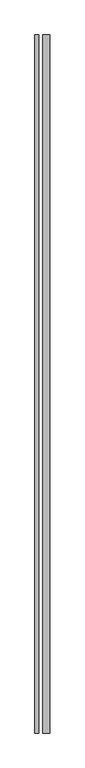
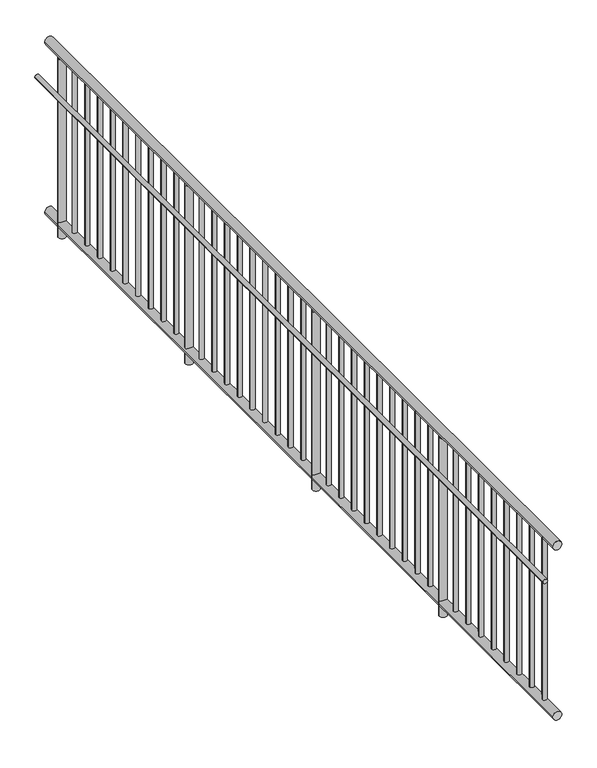
"""IFC4 building model written with IfcOpenShell, lengths in millimetres: railing geometry."""

from ifc_helpers import new_model, si_unit, point, frame, frame_2d, origin, place, context, project, spatial, circle_curve, trimmed, segment, composite_curve, outline, extrude, source, transform, mapped, element, save


def railing_ee1e5d7c(model_context):
    return source(origin(), model_context, "Body", "SweptSolid", [
        extrude(outline(composite_curve([segment(trimmed(circle_curve(frame_2d((4474.6, -1025.274449)), 25.4), [point((4474.6, -999.874449))], [point((4474.6, -1050.674449))], False, "CARTESIAN"), True, "CONTINUOUS"), segment(trimmed(circle_curve(frame_2d((4474.6, -1025.274449)), 25.4), [point((4474.6, -1050.674449))], [point((4474.6, -999.874449))], False, "CARTESIAN"), True, "CONTINUOUS")], self_intersect=False)), frame((0.0, -6784.1965465, 0.0), z_axis=(0.0, 1.0, 0.0), x_axis=(0.0, 0.0, 1.0)), (0.0, 0.0, 1.0), 4890.8),
        extrude(outline(composite_curve([segment(trimmed(circle_curve(frame_2d((4287.3, -1092.274449)), 12.7), [point((4287.3, -1079.574449))], [point((4287.3, -1104.974449))], False, "CARTESIAN"), True, "CONTINUOUS"), segment(trimmed(circle_curve(frame_2d((4287.3, -1092.274449)), 12.7), [point((4287.3, -1104.974449))], [point((4287.3, -1079.574449))], False, "CARTESIAN"), True, "CONTINUOUS")], self_intersect=False)), frame((0.0, -6784.1965465, 0.0), z_axis=(0.0, 1.0, 0.0), x_axis=(0.0, 0.0, 1.0)), (0.0, 0.0, 1.0), 4890.8),
        extrude(outline(composite_curve([segment(trimmed(circle_curve(frame_2d((3474.6, -1025.274449)), 25.4), [point((3474.6, -999.874449))], [point((3474.6, -1050.674449))], False, "CARTESIAN"), True, "CONTINUOUS"), segment(trimmed(circle_curve(frame_2d((3474.6, -1025.274449)), 25.4), [point((3474.6, -1050.674449))], [point((3474.6, -999.874449))], False, "CARTESIAN"), True, "CONTINUOUS")], self_intersect=False)), frame((0.0, -6784.1965465, 0.0), z_axis=(0.0, 1.0, 0.0), x_axis=(0.0, 0.0, 1.0)), (0.0, 0.0, 1.0), 4890.8),
        extrude(outline(composite_curve([segment(trimmed(circle_curve(frame_2d((-1025.274449, -6661.9265465)), 12.5), [point((-1012.774449, -6661.9265465))], [point((-1037.774449, -6661.9265465))], False, "CARTESIAN"), True, "CONTINUOUS"), segment(trimmed(circle_curve(frame_2d((-1025.274449, -6661.9265465)), 12.5), [point((-1037.774449, -6661.9265465))], [point((-1012.774449, -6661.9265465))], False, "CARTESIAN"), True, "CONTINUOUS")], self_intersect=False)), frame((0.0, 0.0, 3500.0), z_axis=(0.0, 0.0, 1.0), x_axis=(1.0, 0.0, 0.0)), (0.0, 0.0, 1.0), 949.2),
        extrude(outline(composite_curve([segment(trimmed(circle_curve(frame_2d((-1025.274449, -6539.6565465)), 12.5), [point((-1012.774449, -6539.6565465))], [point((-1037.774449, -6539.6565465))], False, "CARTESIAN"), True, "CONTINUOUS"), segment(trimmed(circle_curve(frame_2d((-1025.274449, -6539.6565465)), 12.5), [point((-1037.774449, -6539.6565465))], [point((-1012.774449, -6539.6565465))], False, "CARTESIAN"), True, "CONTINUOUS")], self_intersect=False)), frame((0.0, 0.0, 3500.0), z_axis=(0.0, 0.0, 1.0), x_axis=(1.0, 0.0, 0.0)), (0.0, 0.0, 1.0), 949.2),
        extrude(outline(composite_curve([segment(trimmed(circle_curve(frame_2d((-1025.274449, -6417.3865465)), 12.5), [point((-1012.774449, -6417.3865465))], [point((-1037.774449, -6417.3865465))], False, "CARTESIAN"), True, "CONTINUOUS"), segment(trimmed(circle_curve(frame_2d((-1025.274449, -6417.3865465)), 12.5), [point((-1037.774449, -6417.3865465))], [point((-1012.774449, -6417.3865465))], False, "CARTESIAN"), True, "CONTINUOUS")], self_intersect=False)), frame((0.0, 0.0, 3500.0), z_axis=(0.0, 0.0, 1.0), x_axis=(1.0, 0.0, 0.0)), (0.0, 0.0, 1.0), 949.2),
        extrude(outline(composite_curve([segment(trimmed(circle_curve(frame_2d((-1025.274449, -6295.1165465)), 12.5), [point((-1012.774449, -6295.1165465))], [point((-1037.774449, -6295.1165465))], False, "CARTESIAN"), True, "CONTINUOUS"), segment(trimmed(circle_curve(frame_2d((-1025.274449, -6295.1165465)), 12.5), [point((-1037.774449, -6295.1165465))], [point((-1012.774449, -6295.1165465))], False, "CARTESIAN"), True, "CONTINUOUS")], self_intersect=False)), frame((0.0, 0.0, 3500.0), z_axis=(0.0, 0.0, 1.0), x_axis=(1.0, 0.0, 0.0)), (0.0, 0.0, 1.0), 949.2),
        extrude(outline(composite_curve([segment(trimmed(circle_curve(frame_2d((-1025.274449, -6172.8465465)), 12.5), [point((-1012.774449, -6172.8465465))], [point((-1037.774449, -6172.8465465))], False, "CARTESIAN"), True, "CONTINUOUS"), segment(trimmed(circle_curve(frame_2d((-1025.274449, -6172.8465465)), 12.5), [point((-1037.774449, -6172.8465465))], [point((-1012.774449, -6172.8465465))], False, "CARTESIAN"), True, "CONTINUOUS")], self_intersect=False)), frame((0.0, 0.0, 3500.0), z_axis=(0.0, 0.0, 1.0), x_axis=(1.0, 0.0, 0.0)), (0.0, 0.0, 1.0), 949.2),
        extrude(outline(composite_curve([segment(trimmed(circle_curve(frame_2d((-1025.274449, -6050.5765465)), 12.5), [point((-1012.774449, -6050.5765465))], [point((-1037.774449, -6050.5765465))], False, "CARTESIAN"), True, "CONTINUOUS"), segment(trimmed(circle_curve(frame_2d((-1025.274449, -6050.5765465)), 12.5), [point((-1037.774449, -6050.5765465))], [point((-1012.774449, -6050.5765465))], False, "CARTESIAN"), True, "CONTINUOUS")], self_intersect=False)), frame((0.0, 0.0, 3500.0), z_axis=(0.0, 0.0, 1.0), x_axis=(1.0, 0.0, 0.0)), (0.0, 0.0, 1.0), 949.2),
        extrude(outline(composite_curve([segment(trimmed(circle_curve(frame_2d((-1025.274449, -5928.3065465)), 12.5), [point((-1012.774449, -5928.3065465))], [point((-1037.774449, -5928.3065465))], False, "CARTESIAN"), True, "CONTINUOUS"), segment(trimmed(circle_curve(frame_2d((-1025.274449, -5928.3065465)), 12.5), [point((-1037.774449, -5928.3065465))], [point((-1012.774449, -5928.3065465))], False, "CARTESIAN"), True, "CONTINUOUS")], self_intersect=False)), frame((0.0, 0.0, 3500.0), z_axis=(0.0, 0.0, 1.0), x_axis=(1.0, 0.0, 0.0)), (0.0, 0.0, 1.0), 949.2),
        extrude(outline(composite_curve([segment(trimmed(circle_curve(frame_2d((-1025.274449, -5806.0365465)), 12.5), [point((-1012.774449, -5806.0365465))], [point((-1037.774449, -5806.0365465))], False, "CARTESIAN"), True, "CONTINUOUS"), segment(trimmed(circle_curve(frame_2d((-1025.274449, -5806.0365465)), 12.5), [point((-1037.774449, -5806.0365465))], [point((-1012.774449, -5806.0365465))], False, "CARTESIAN"), True, "CONTINUOUS")], self_intersect=False)), frame((0.0, 0.0, 3500.0), z_axis=(0.0, 0.0, 1.0), x_axis=(1.0, 0.0, 0.0)), (0.0, 0.0, 1.0), 949.2),
        extrude(outline(composite_curve([segment(trimmed(circle_curve(frame_2d((-1025.274449, -5683.7665465)), 21.0), [point((-1004.274449, -5683.7665465))], [point((-1046.274449, -5683.7665465))], False, "CARTESIAN"), True, "CONTINUOUS"), segment(trimmed(circle_curve(frame_2d((-1025.274449, -5683.7665465)), 21.0), [point((-1046.274449, -5683.7665465))], [point((-1004.274449, -5683.7665465))], False, "CARTESIAN"), True, "CONTINUOUS")], self_intersect=False)), frame((0.0, 0.0, 3400.0), z_axis=(0.0, 0.0, 1.0), x_axis=(1.0, 0.0, 0.0)), (0.0, 0.0, 1.0), 1049.2),
        extrude(outline(composite_curve([segment(trimmed(circle_curve(frame_2d((-1025.274449, -5561.4965465)), 12.5), [point((-1012.774449, -5561.4965465))], [point((-1037.774449, -5561.4965465))], False, "CARTESIAN"), True, "CONTINUOUS"), segment(trimmed(circle_curve(frame_2d((-1025.274449, -5561.4965465)), 12.5), [point((-1037.774449, -5561.4965465))], [point((-1012.774449, -5561.4965465))], False, "CARTESIAN"), True, "CONTINUOUS")], self_intersect=False)), frame((0.0, 0.0, 3500.0), z_axis=(0.0, 0.0, 1.0), x_axis=(1.0, 0.0, 0.0)), (0.0, 0.0, 1.0), 949.2),
        extrude(outline(composite_curve([segment(trimmed(circle_curve(frame_2d((-1025.274449, -5439.2265465)), 12.5), [point((-1012.774449, -5439.2265465))], [point((-1037.774449, -5439.2265465))], False, "CARTESIAN"), True, "CONTINUOUS"), segment(trimmed(circle_curve(frame_2d((-1025.274449, -5439.2265465)), 12.5), [point((-1037.774449, -5439.2265465))], [point((-1012.774449, -5439.2265465))], False, "CARTESIAN"), True, "CONTINUOUS")], self_intersect=False)), frame((0.0, 0.0, 3500.0), z_axis=(0.0, 0.0, 1.0), x_axis=(1.0, 0.0, 0.0)), (0.0, 0.0, 1.0), 949.2),
        extrude(outline(composite_curve([segment(trimmed(circle_curve(frame_2d((-1025.274449, -5316.9565465)), 12.5), [point((-1012.774449, -5316.9565465))], [point((-1037.774449, -5316.9565465))], False, "CARTESIAN"), True, "CONTINUOUS"), segment(trimmed(circle_curve(frame_2d((-1025.274449, -5316.9565465)), 12.5), [point((-1037.774449, -5316.9565465))], [point((-1012.774449, -5316.9565465))], False, "CARTESIAN"), True, "CONTINUOUS")], self_intersect=False)), frame((0.0, 0.0, 3500.0), z_axis=(0.0, 0.0, 1.0), x_axis=(1.0, 0.0, 0.0)), (0.0, 0.0, 1.0), 949.2),
        extrude(outline(composite_curve([segment(trimmed(circle_curve(frame_2d((-1025.274449, -5194.6865465)), 12.5), [point((-1012.774449, -5194.6865465))], [point((-1037.774449, -5194.6865465))], False, "CARTESIAN"), True, "CONTINUOUS"), segment(trimmed(circle_curve(frame_2d((-1025.274449, -5194.6865465)), 12.5), [point((-1037.774449, -5194.6865465))], [point((-1012.774449, -5194.6865465))], False, "CARTESIAN"), True, "CONTINUOUS")], self_intersect=False)), frame((0.0, 0.0, 3500.0), z_axis=(0.0, 0.0, 1.0), x_axis=(1.0, 0.0, 0.0)), (0.0, 0.0, 1.0), 949.2),
        extrude(outline(composite_curve([segment(trimmed(circle_curve(frame_2d((-1025.274449, -5072.4165465)), 12.5), [point((-1012.774449, -5072.4165465))], [point((-1037.774449, -5072.4165465))], False, "CARTESIAN"), True, "CONTINUOUS"), segment(trimmed(circle_curve(frame_2d((-1025.274449, -5072.4165465)), 12.5), [point((-1037.774449, -5072.4165465))], [point((-1012.774449, -5072.4165465))], False, "CARTESIAN"), True, "CONTINUOUS")], self_intersect=False)), frame((0.0, 0.0, 3500.0), z_axis=(0.0, 0.0, 1.0), x_axis=(1.0, 0.0, 0.0)), (0.0, 0.0, 1.0), 949.2),
        extrude(outline(composite_curve([segment(trimmed(circle_curve(frame_2d((-1025.274449, -4950.1465465)), 12.5), [point((-1012.774449, -4950.1465465))], [point((-1037.774449, -4950.1465465))], False, "CARTESIAN"), True, "CONTINUOUS"), segment(trimmed(circle_curve(frame_2d((-1025.274449, -4950.1465465)), 12.5), [point((-1037.774449, -4950.1465465))], [point((-1012.774449, -4950.1465465))], False, "CARTESIAN"), True, "CONTINUOUS")], self_intersect=False)), frame((0.0, 0.0, 3500.0), z_axis=(0.0, 0.0, 1.0), x_axis=(1.0, 0.0, 0.0)), (0.0, 0.0, 1.0), 949.2),
        extrude(outline(composite_curve([segment(trimmed(circle_curve(frame_2d((-1025.274449, -4827.8765465)), 12.5), [point((-1012.774449, -4827.8765465))], [point((-1037.774449, -4827.8765465))], False, "CARTESIAN"), True, "CONTINUOUS"), segment(trimmed(circle_curve(frame_2d((-1025.274449, -4827.8765465)), 12.5), [point((-1037.774449, -4827.8765465))], [point((-1012.774449, -4827.8765465))], False, "CARTESIAN"), True, "CONTINUOUS")], self_intersect=False)), frame((0.0, 0.0, 3500.0), z_axis=(0.0, 0.0, 1.0), x_axis=(1.0, 0.0, 0.0)), (0.0, 0.0, 1.0), 949.2),
        extrude(outline(composite_curve([segment(trimmed(circle_curve(frame_2d((-1025.274449, -4705.6065465)), 12.5), [point((-1012.774449, -4705.6065465))], [point((-1037.774449, -4705.6065465))], False, "CARTESIAN"), True, "CONTINUOUS"), segment(trimmed(circle_curve(frame_2d((-1025.274449, -4705.6065465)), 12.5), [point((-1037.774449, -4705.6065465))], [point((-1012.774449, -4705.6065465))], False, "CARTESIAN"), True, "CONTINUOUS")], self_intersect=False)), frame((0.0, 0.0, 3500.0), z_axis=(0.0, 0.0, 1.0), x_axis=(1.0, 0.0, 0.0)), (0.0, 0.0, 1.0), 949.2),
        extrude(outline(composite_curve([segment(trimmed(circle_curve(frame_2d((-1025.274449, -4583.3365465)), 12.5), [point((-1012.774449, -4583.3365465))], [point((-1037.774449, -4583.3365465))], False, "CARTESIAN"), True, "CONTINUOUS"), segment(trimmed(circle_curve(frame_2d((-1025.274449, -4583.3365465)), 12.5), [point((-1037.774449, -4583.3365465))], [point((-1012.774449, -4583.3365465))], False, "CARTESIAN"), True, "CONTINUOUS")], self_intersect=False)), frame((0.0, 0.0, 3500.0), z_axis=(0.0, 0.0, 1.0), x_axis=(1.0, 0.0, 0.0)), (0.0, 0.0, 1.0), 949.2),
        extrude(outline(composite_curve([segment(trimmed(circle_curve(frame_2d((-1025.274449, -4461.0665465)), 21.0), [point((-1004.274449, -4461.0665465))], [point((-1046.274449, -4461.0665465))], False, "CARTESIAN"), True, "CONTINUOUS"), segment(trimmed(circle_curve(frame_2d((-1025.274449, -4461.0665465)), 21.0), [point((-1046.274449, -4461.0665465))], [point((-1004.274449, -4461.0665465))], False, "CARTESIAN"), True, "CONTINUOUS")], self_intersect=False)), frame((0.0, 0.0, 3400.0), z_axis=(0.0, 0.0, 1.0), x_axis=(1.0, 0.0, 0.0)), (0.0, 0.0, 1.0), 1049.2),
        extrude(outline(composite_curve([segment(trimmed(circle_curve(frame_2d((-1025.274449, -4338.7965465)), 12.5), [point((-1012.774449, -4338.7965465))], [point((-1037.774449, -4338.7965465))], False, "CARTESIAN"), True, "CONTINUOUS"), segment(trimmed(circle_curve(frame_2d((-1025.274449, -4338.7965465)), 12.5), [point((-1037.774449, -4338.7965465))], [point((-1012.774449, -4338.7965465))], False, "CARTESIAN"), True, "CONTINUOUS")], self_intersect=False)), frame((0.0, 0.0, 3500.0), z_axis=(0.0, 0.0, 1.0), x_axis=(1.0, 0.0, 0.0)), (0.0, 0.0, 1.0), 949.2),
        extrude(outline(composite_curve([segment(trimmed(circle_curve(frame_2d((-1025.274449, -4216.5265465)), 12.5), [point((-1012.774449, -4216.5265465))], [point((-1037.774449, -4216.5265465))], False, "CARTESIAN"), True, "CONTINUOUS"), segment(trimmed(circle_curve(frame_2d((-1025.274449, -4216.5265465)), 12.5), [point((-1037.774449, -4216.5265465))], [point((-1012.774449, -4216.5265465))], False, "CARTESIAN"), True, "CONTINUOUS")], self_intersect=False)), frame((0.0, 0.0, 3500.0), z_axis=(0.0, 0.0, 1.0), x_axis=(1.0, 0.0, 0.0)), (0.0, 0.0, 1.0), 949.2),
        extrude(outline(composite_curve([segment(trimmed(circle_curve(frame_2d((-1025.274449, -4094.2565465)), 12.5), [point((-1012.774449, -4094.2565465))], [point((-1037.774449, -4094.2565465))], False, "CARTESIAN"), True, "CONTINUOUS"), segment(trimmed(circle_curve(frame_2d((-1025.274449, -4094.2565465)), 12.5), [point((-1037.774449, -4094.2565465))], [point((-1012.774449, -4094.2565465))], False, "CARTESIAN"), True, "CONTINUOUS")], self_intersect=False)), frame((0.0, 0.0, 3500.0), z_axis=(0.0, 0.0, 1.0), x_axis=(1.0, 0.0, 0.0)), (0.0, 0.0, 1.0), 949.2),
        extrude(outline(composite_curve([segment(trimmed(circle_curve(frame_2d((-1025.274449, -3971.9865465)), 12.5), [point((-1012.774449, -3971.9865465))], [point((-1037.774449, -3971.9865465))], False, "CARTESIAN"), True, "CONTINUOUS"), segment(trimmed(circle_curve(frame_2d((-1025.274449, -3971.9865465)), 12.5), [point((-1037.774449, -3971.9865465))], [point((-1012.774449, -3971.9865465))], False, "CARTESIAN"), True, "CONTINUOUS")], self_intersect=False)), frame((0.0, 0.0, 3500.0), z_axis=(0.0, 0.0, 1.0), x_axis=(1.0, 0.0, 0.0)), (0.0, 0.0, 1.0), 949.2),
        extrude(outline(composite_curve([segment(trimmed(circle_curve(frame_2d((-1025.274449, -3849.7165465)), 12.5), [point((-1012.774449, -3849.7165465))], [point((-1037.774449, -3849.7165465))], False, "CARTESIAN"), True, "CONTINUOUS"), segment(trimmed(circle_curve(frame_2d((-1025.274449, -3849.7165465)), 12.5), [point((-1037.774449, -3849.7165465))], [point((-1012.774449, -3849.7165465))], False, "CARTESIAN"), True, "CONTINUOUS")], self_intersect=False)), frame((0.0, 0.0, 3500.0), z_axis=(0.0, 0.0, 1.0), x_axis=(1.0, 0.0, 0.0)), (0.0, 0.0, 1.0), 949.2),
        extrude(outline(composite_curve([segment(trimmed(circle_curve(frame_2d((-1025.274449, -3727.4465465)), 12.5), [point((-1012.774449, -3727.4465465))], [point((-1037.774449, -3727.4465465))], False, "CARTESIAN"), True, "CONTINUOUS"), segment(trimmed(circle_curve(frame_2d((-1025.274449, -3727.4465465)), 12.5), [point((-1037.774449, -3727.4465465))], [point((-1012.774449, -3727.4465465))], False, "CARTESIAN"), True, "CONTINUOUS")], self_intersect=False)), frame((0.0, 0.0, 3500.0), z_axis=(0.0, 0.0, 1.0), x_axis=(1.0, 0.0, 0.0)), (0.0, 0.0, 1.0), 949.2),
        extrude(outline(composite_curve([segment(trimmed(circle_curve(frame_2d((-1025.274449, -3605.1765465)), 12.5), [point((-1012.774449, -3605.1765465))], [point((-1037.774449, -3605.1765465))], False, "CARTESIAN"), True, "CONTINUOUS"), segment(trimmed(circle_curve(frame_2d((-1025.274449, -3605.1765465)), 12.5), [point((-1037.774449, -3605.1765465))], [point((-1012.774449, -3605.1765465))], False, "CARTESIAN"), True, "CONTINUOUS")], self_intersect=False)), frame((0.0, 0.0, 3500.0), z_axis=(0.0, 0.0, 1.0), x_axis=(1.0, 0.0, 0.0)), (0.0, 0.0, 1.0), 949.2),
        extrude(outline(composite_curve([segment(trimmed(circle_curve(frame_2d((-1025.274449, -3482.9065465)), 12.5), [point((-1012.774449, -3482.9065465))], [point((-1037.774449, -3482.9065465))], False, "CARTESIAN"), True, "CONTINUOUS"), segment(trimmed(circle_curve(frame_2d((-1025.274449, -3482.9065465)), 12.5), [point((-1037.774449, -3482.9065465))], [point((-1012.774449, -3482.9065465))], False, "CARTESIAN"), True, "CONTINUOUS")], self_intersect=False)), frame((0.0, 0.0, 3500.0), z_axis=(0.0, 0.0, 1.0), x_axis=(1.0, 0.0, 0.0)), (0.0, 0.0, 1.0), 949.2),
        extrude(outline(composite_curve([segment(trimmed(circle_curve(frame_2d((-1025.274449, -3360.6365465)), 12.5), [point((-1012.774449, -3360.6365465))], [point((-1037.774449, -3360.6365465))], False, "CARTESIAN"), True, "CONTINUOUS"), segment(trimmed(circle_curve(frame_2d((-1025.274449, -3360.6365465)), 12.5), [point((-1037.774449, -3360.6365465))], [point((-1012.774449, -3360.6365465))], False, "CARTESIAN"), True, "CONTINUOUS")], self_intersect=False)), frame((0.0, 0.0, 3500.0), z_axis=(0.0, 0.0, 1.0), x_axis=(1.0, 0.0, 0.0)), (0.0, 0.0, 1.0), 949.2),
        extrude(outline(composite_curve([segment(trimmed(circle_curve(frame_2d((-1025.274449, -3238.3665465)), 21.0), [point((-1004.274449, -3238.3665465))], [point((-1046.274449, -3238.3665465))], False, "CARTESIAN"), True, "CONTINUOUS"), segment(trimmed(circle_curve(frame_2d((-1025.274449, -3238.3665465)), 21.0), [point((-1046.274449, -3238.3665465))], [point((-1004.274449, -3238.3665465))], False, "CARTESIAN"), True, "CONTINUOUS")], self_intersect=False)), frame((0.0, 0.0, 3400.0), z_axis=(0.0, 0.0, 1.0), x_axis=(1.0, 0.0, 0.0)), (0.0, 0.0, 1.0), 1049.2),
        extrude(outline(composite_curve([segment(trimmed(circle_curve(frame_2d((-1025.274449, -3116.0965465)), 12.5), [point((-1012.774449, -3116.0965465))], [point((-1037.774449, -3116.0965465))], False, "CARTESIAN"), True, "CONTINUOUS"), segment(trimmed(circle_curve(frame_2d((-1025.274449, -3116.0965465)), 12.5), [point((-1037.774449, -3116.0965465))], [point((-1012.774449, -3116.0965465))], False, "CARTESIAN"), True, "CONTINUOUS")], self_intersect=False)), frame((0.0, 0.0, 3500.0), z_axis=(0.0, 0.0, 1.0), x_axis=(1.0, 0.0, 0.0)), (0.0, 0.0, 1.0), 949.2),
        extrude(outline(composite_curve([segment(trimmed(circle_curve(frame_2d((-1025.274449, -2993.8265465)), 12.5), [point((-1012.774449, -2993.8265465))], [point((-1037.774449, -2993.8265465))], False, "CARTESIAN"), True, "CONTINUOUS"), segment(trimmed(circle_curve(frame_2d((-1025.274449, -2993.8265465)), 12.5), [point((-1037.774449, -2993.8265465))], [point((-1012.774449, -2993.8265465))], False, "CARTESIAN"), True, "CONTINUOUS")], self_intersect=False)), frame((0.0, 0.0, 3500.0), z_axis=(0.0, 0.0, 1.0), x_axis=(1.0, 0.0, 0.0)), (0.0, 0.0, 1.0), 949.2),
        extrude(outline(composite_curve([segment(trimmed(circle_curve(frame_2d((-1025.274449, -2871.5565465)), 12.5), [point((-1012.774449, -2871.5565465))], [point((-1037.774449, -2871.5565465))], False, "CARTESIAN"), True, "CONTINUOUS"), segment(trimmed(circle_curve(frame_2d((-1025.274449, -2871.5565465)), 12.5), [point((-1037.774449, -2871.5565465))], [point((-1012.774449, -2871.5565465))], False, "CARTESIAN"), True, "CONTINUOUS")], self_intersect=False)), frame((0.0, 0.0, 3500.0), z_axis=(0.0, 0.0, 1.0), x_axis=(1.0, 0.0, 0.0)), (0.0, 0.0, 1.0), 949.2),
        extrude(outline(composite_curve([segment(trimmed(circle_curve(frame_2d((-1025.274449, -2749.2865465)), 12.5), [point((-1012.774449, -2749.2865465))], [point((-1037.774449, -2749.2865465))], False, "CARTESIAN"), True, "CONTINUOUS"), segment(trimmed(circle_curve(frame_2d((-1025.274449, -2749.2865465)), 12.5), [point((-1037.774449, -2749.2865465))], [point((-1012.774449, -2749.2865465))], False, "CARTESIAN"), True, "CONTINUOUS")], self_intersect=False)), frame((0.0, 0.0, 3500.0), z_axis=(0.0, 0.0, 1.0), x_axis=(1.0, 0.0, 0.0)), (0.0, 0.0, 1.0), 949.2),
        extrude(outline(composite_curve([segment(trimmed(circle_curve(frame_2d((-1025.274449, -2627.0165465)), 12.5), [point((-1012.774449, -2627.0165465))], [point((-1037.774449, -2627.0165465))], False, "CARTESIAN"), True, "CONTINUOUS"), segment(trimmed(circle_curve(frame_2d((-1025.274449, -2627.0165465)), 12.5), [point((-1037.774449, -2627.0165465))], [point((-1012.774449, -2627.0165465))], False, "CARTESIAN"), True, "CONTINUOUS")], self_intersect=False)), frame((0.0, 0.0, 3500.0), z_axis=(0.0, 0.0, 1.0), x_axis=(1.0, 0.0, 0.0)), (0.0, 0.0, 1.0), 949.2),
        extrude(outline(composite_curve([segment(trimmed(circle_curve(frame_2d((-1025.274449, -2504.7465465)), 12.5), [point((-1012.774449, -2504.7465465))], [point((-1037.774449, -2504.7465465))], False, "CARTESIAN"), True, "CONTINUOUS"), segment(trimmed(circle_curve(frame_2d((-1025.274449, -2504.7465465)), 12.5), [point((-1037.774449, -2504.7465465))], [point((-1012.774449, -2504.7465465))], False, "CARTESIAN"), True, "CONTINUOUS")], self_intersect=False)), frame((0.0, 0.0, 3500.0), z_axis=(0.0, 0.0, 1.0), x_axis=(1.0, 0.0, 0.0)), (0.0, 0.0, 1.0), 949.2),
        extrude(outline(composite_curve([segment(trimmed(circle_curve(frame_2d((-1025.274449, -2382.4765465)), 12.5), [point((-1012.774449, -2382.4765465))], [point((-1037.774449, -2382.4765465))], False, "CARTESIAN"), True, "CONTINUOUS"), segment(trimmed(circle_curve(frame_2d((-1025.274449, -2382.4765465)), 12.5), [point((-1037.774449, -2382.4765465))], [point((-1012.774449, -2382.4765465))], False, "CARTESIAN"), True, "CONTINUOUS")], self_intersect=False)), frame((0.0, 0.0, 3500.0), z_axis=(0.0, 0.0, 1.0), x_axis=(1.0, 0.0, 0.0)), (0.0, 0.0, 1.0), 949.2),
        extrude(outline(composite_curve([segment(trimmed(circle_curve(frame_2d((-1025.274449, -2260.2065465)), 12.5), [point((-1012.774449, -2260.2065465))], [point((-1037.774449, -2260.2065465))], False, "CARTESIAN"), True, "CONTINUOUS"), segment(trimmed(circle_curve(frame_2d((-1025.274449, -2260.2065465)), 12.5), [point((-1037.774449, -2260.2065465))], [point((-1012.774449, -2260.2065465))], False, "CARTESIAN"), True, "CONTINUOUS")], self_intersect=False)), frame((0.0, 0.0, 3500.0), z_axis=(0.0, 0.0, 1.0), x_axis=(1.0, 0.0, 0.0)), (0.0, 0.0, 1.0), 949.2),
        extrude(outline(composite_curve([segment(trimmed(circle_curve(frame_2d((-1025.274449, -2137.9365465)), 12.5), [point((-1012.774449, -2137.9365465))], [point((-1037.774449, -2137.9365465))], False, "CARTESIAN"), True, "CONTINUOUS"), segment(trimmed(circle_curve(frame_2d((-1025.274449, -2137.9365465)), 12.5), [point((-1037.774449, -2137.9365465))], [point((-1012.774449, -2137.9365465))], False, "CARTESIAN"), True, "CONTINUOUS")], self_intersect=False)), frame((0.0, 0.0, 3500.0), z_axis=(0.0, 0.0, 1.0), x_axis=(1.0, 0.0, 0.0)), (0.0, 0.0, 1.0), 949.2),
        extrude(outline(composite_curve([segment(trimmed(circle_curve(frame_2d((-1025.274449, -2015.6665465)), 21.0), [point((-1004.274449, -2015.6665465))], [point((-1046.274449, -2015.6665465))], False, "CARTESIAN"), True, "CONTINUOUS"), segment(trimmed(circle_curve(frame_2d((-1025.274449, -2015.6665465)), 21.0), [point((-1046.274449, -2015.6665465))], [point((-1004.274449, -2015.6665465))], False, "CARTESIAN"), True, "CONTINUOUS")], self_intersect=False)), frame((0.0, 0.0, 3400.0), z_axis=(0.0, 0.0, 1.0), x_axis=(1.0, 0.0, 0.0)), (0.0, 0.0, 1.0), 1049.2),
    ])


if __name__ == "__main__":
    model = new_model("IFC4")
    model_context = context("Model", 3, world=origin())
    ifc_project = project(units=[si_unit("LENGTHUNIT", "METRE", prefix="MILLI")], contexts=[model_context])
    site = spatial("IfcSite", under=ifc_project)
    building = spatial("IfcBuilding", under=site)
    placement = place(None, origin())
    railing_shape = railing_ee1e5d7c(model_context)
    element("IfcRailing", 1, at=placement, inside=building, context=model_context, shape_type="MappedRepresentation", body=[
        mapped(railing_shape, transform((0.0, 0.0, 0.0), x_axis=(1.0, 0.0, 0.0), y_axis=(0.0, 1.0, 0.0), z_axis=(0.0, 0.0, 1.0))),
    ])
    save(model, "model.ifc")

# Revit data of these elements
# Element 1 (IfcRailing)
#   Materials on its faces: "Ferro - Pintura Esmalte"
# Materials
#   "Ferro - Pintura Esmalte": class "Pintura", colour RGB 255 255 255, transparency 0, Cost = 0
